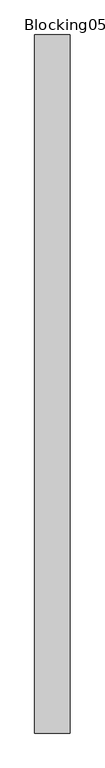
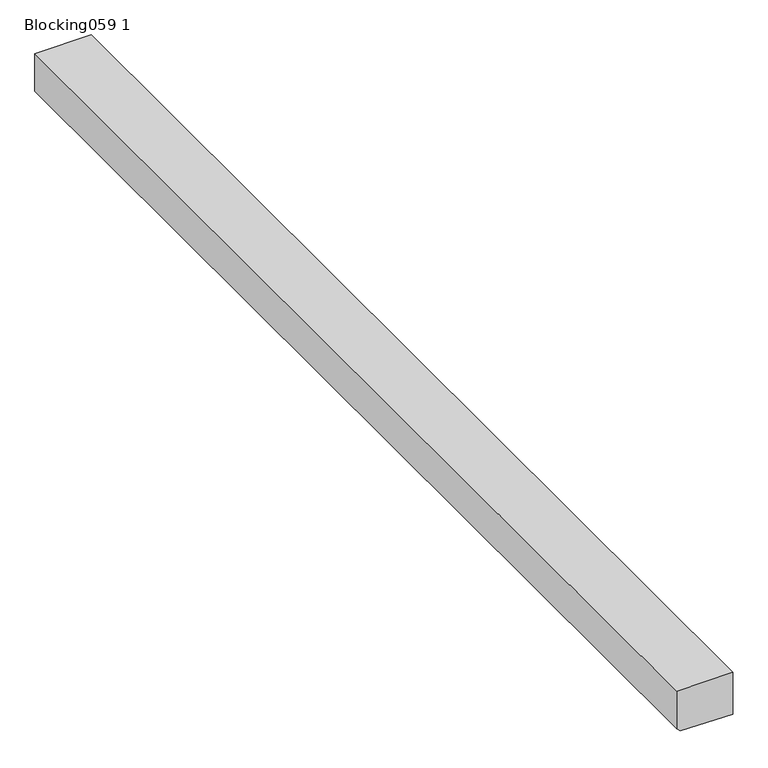
"""IFC4 building model written with IfcOpenShell, lengths in millimetres: proxy geometry, Blocking059 1 : Blocking059 1918."""

from ifc_helpers import new_model, si_unit, frame, origin, place, context, project, spatial, polyline, outline, extrude, source, transform, mapped, element, save


def blocking059_1_d2a3d8a8(model_context):
    return source(origin(), model_context, "Body", "SweptSolid", [
        extrude(outline(polyline([(40118.3092895, -7012.6070533), (40118.3092895, -7114.2070533), (40047.0174737, -7114.2070533), (40040.2769302, -7107.5750792), (40038.291814, -7012.6070533), (40118.3092895, -7012.6070533)])), frame((0.0, 7182.1531721, 0.0), z_axis=(0.0, 1.0, 0.0), x_axis=(0.0, 0.0, 1.0)), (0.0, 0.0, 1.0), 2000.0),
    ])


if __name__ == "__main__":
    model = new_model("IFC4")
    model_context = context("Model", 3, world=origin())
    ifc_project = project(units=[si_unit("LENGTHUNIT", "METRE", prefix="MILLI")], contexts=[model_context])
    site = spatial("IfcSite", under=ifc_project)
    building = spatial("IfcBuilding", under=site)
    placement = place(None, origin())
    blocking059_1_shape = blocking059_1_d2a3d8a8(model_context)
    element("IfcBuildingElementProxy", 1, Name="Blocking059 1 : Blocking059 1918", ObjectType="Blocking059 1 : Blocking059 1918", at=placement, inside=building, context=model_context, shape_type="MappedRepresentation", body=[
        mapped(blocking059_1_shape, transform((0.0, 0.0, 0.0), x_axis=(1.0, 0.0, 0.0), y_axis=(0.0, 1.0, 0.0), z_axis=(0.0, 0.0, 1.0))),
    ])
    save(model, "model.ifc")

# Revit data of these elements
# Type "Blocking059 1 : Blocking059 1918"
#   NameOverride = "Blocking059"
# Element 1 (IfcBuildingElementProxy, "Blocking059 1 : Blocking059 1918")
#   Materials on its faces: "TREATED INTERMITTENT (FOR DRAINAGE) BLOCKING - SET IN BED OF SEALANT"
# Materials
#   "TREATED INTERMITTENT (FOR DRAINAGE) BLOCKING - SET IN BED OF SEALANT": class "Unassigned", colour RGB 140 161 107, transparency 0, Cost = 0
